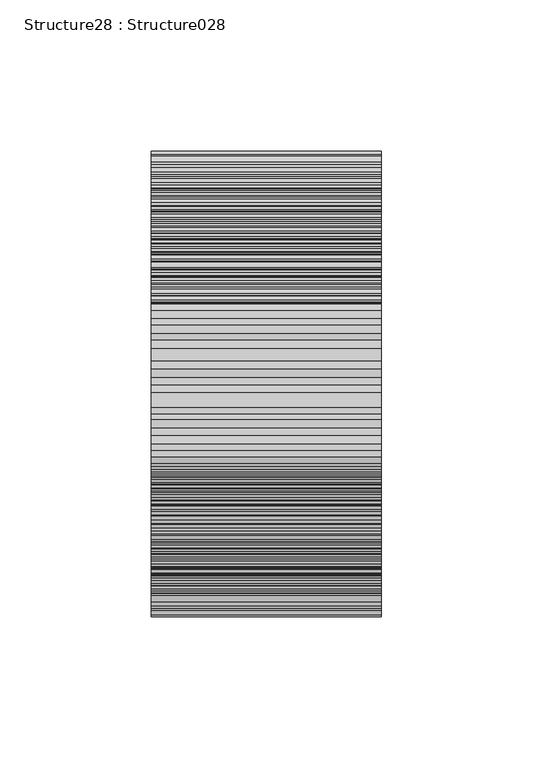
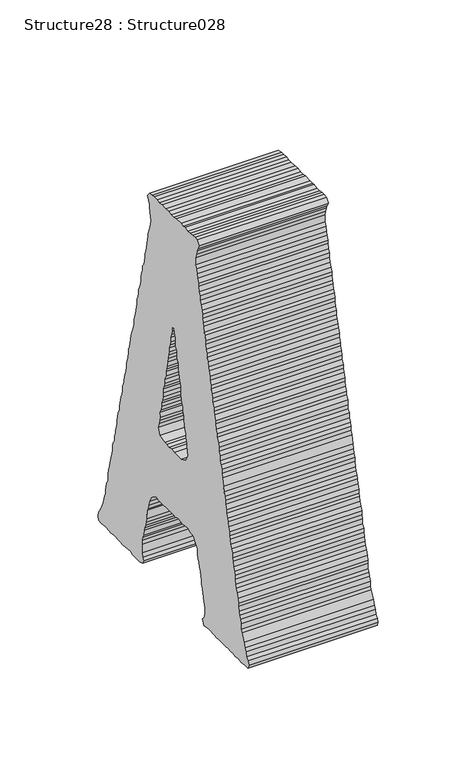
"""IFC4 building model written with IfcOpenShell, lengths in millimetres: proxy geometry, Structure28 : Structure028."""

from ifc_helpers import new_model, si_unit, frame, origin, place, context, project, spatial, polyline, outline, extrude, source, transform, mapped, element, save


def structure28_structure028_1b6d3d0a(model_context):
    return source(origin(), model_context, "Body", "SweptSolid", [
        extrude(outline(polyline([(2.1653931, 0.0), (4.9551582, -1.2360362), (7.1205514, -1.5537289), (9.8959144, -1.859561), (12.3790002, -2.7770574), (14.2258535, -3.09475), (17.0249376, -4.024107), (19.4987044, -4.024107), (22.2740675, -4.9543111), (24.4394606, -5.5778358), (27.2292257, -6.1895001), (29.3937717, -6.8011644), (31.8616083, -7.1069965), (33.7101559, -8.0372006), (36.8159193, -8.3548933), (38.9813125, -8.3548933), (41.7583699, -8.978418), (43.3112516, -9.907775), (46.4093904, -10.5075787), (48.2664099, -11.1311035), (50.7384823, -11.7546283), (53.207166, -11.7546283), (55.371712, -12.3790002), (58.1614771, -13.3083572), (60.6428686, -14.2258535), (63.419926, -14.2258535), (65.2676265, -15.1552105), (68.3750842, -15.7787352), (70.2219375, -15.7787352), (72.7041762, -16.7089393), (75.1770958, -17.0147715), (77.9524588, -17.6382963), (80.1322541, -18.5557927), (84.4621932, -18.5557927), (86.9291825, -17.9441284), (89.4029494, -17.3324641), (91.2591217, -16.3912467), (93.7311941, -15.1552105), (96.2142799, -17.3324641), (96.5226536, -19.4851496), (96.5226536, -21.6624032), (95.9109893, -24.4394606), (95.9109893, -26.9098387), (96.5226536, -29.6987567), (96.2142799, -31.5574705), (96.5226536, -33.7228637), (96.5226536, -38.664467), (95.9109893, -41.1475528), (95.9109893, -43.6187781), (96.5226536, -46.3949883), (96.2142799, -49.1957668), (96.2142799, -53.2080132), (95.9109893, -55.9969312), (96.5226536, -58.1496166), (96.5226536, -60.9503951), (96.2142799, -63.1039277), (95.9109893, -65.8801379), (93.4245148, -67.7515595), (91.2591217, -66.5036627), (89.0945757, -65.8801379), (87.2375562, -65.5861663), (84.4621932, -64.9626415), (79.8094783, -64.0332846), (77.6457795, -64.6568094), (74.8687221, -65.2803342), (69.9135639, -67.1280347), (68.3750842, -67.1280347), (65.5853191, -67.7515595), (63.1166354, -68.3632237), (60.3268703, -68.6809164), (57.8437845, -69.3044412), (55.371712, -70.5277697), (53.5155397, -70.5277697), (50.7384823, -70.834449), (48.2664099, -71.4579738), (46.4093904, -72.7050234), (43.6196253, -72.7050234), (41.1467056, -73.6225198), (38.9813125, -74.234184), (36.5134759, -74.234184), (33.7101559, -74.858556), (31.2507912, -75.7879129), (29.085398, -76.7172698), (27.2292257, -77.0349625), (24.4394606, -77.3407946), (22.2740675, -78.258291), (19.4987044, -78.258291), (17.0249376, -79.1884951), (14.8510727, -79.5061877), (12.0748624, -80.117852), (7.7322156, -81.6588732), (4.9551582, -81.6588732), (2.7906123, -82.282398), (0.3176926, -82.9067699), (-2.4720725, -84.141959), (-4.3282448, -84.4596516), (-6.8020116, -85.0713159), (-9.283403, -85.3890086), (-12.0604605, -86.306505), (-13.9217158, -86.9308769), (-16.7063979, -86.9308769), (-19.4826081, -87.8602338), (-21.3438635, -88.166066), (-24.1344758, -89.0954229), (-26.5929933, -89.4131155), (-29.0752319, -89.7070871), (-30.9322514, -90.3306119), (-33.4136429, -91.260816), (-36.4982268, -91.5666482), (-38.9711464, -92.1901729), (-40.5240281, -93.1195299), (-43.3002383, -93.1195299), (-46.0908506, -93.7311941), (-48.2553966, -94.6613982), (-51.0409258, -95.284923), (-52.9021812, -95.8965873), (-55.0531722, -96.5201121), (-57.5354109, -96.5201121), (-60.6327025, -97.7434406), (-63.1013862, -98.3678125), (-65.2794871, -98.6855052), (-67.7524067, -98.6855052), (-69.6094262, -99.2971695), (-72.6931629, -100.2265264), (-74.5501824, -100.544219), (-77.032421, -101.4617154), (-79.8128671, -101.4617154), (-81.9782603, -102.6977517), (-84.1428062, -103.3212764), (-86.6106428, -103.3212764), (-89.386853, -103.9448012), (-92.1910202, -104.8741582), (-94.3420113, -105.4858224), (-96.2032666, -106.0983339), (-98.9887958, -106.4160265), (-101.4617155, -107.3453834), (-104.2514806, -107.9689082), (-106.7193172, -107.9689082), (-108.8982652, -108.2747403), (-111.0492563, -109.5099294), (-113.8390214, -110.1224408), (-116.311941, -110.7459656), (-118.476487, -110.7459656), (-120.6503519, -111.6753225), (-125.8994818, -113.2163437), (-128.0784298, -114.1465478), (-129.9261303, -115.0759047), (-132.7116595, -116.9346186), (-134.2560694, -117.5462828), (-137.0314325, -118.4764869), (-139.2061446, -117.8529621), (-139.5136711, -114.7700726), (-139.2061446, -112.9223721), (-138.8884519, -110.1224408), (-139.5136711, -107.6512156), (-139.5136711, -104.8741582), (-138.8884519, -102.3919195), (-138.8884519, -100.2265264), (-139.2061446, -97.7434406), (-139.2061446, -95.5907551), (-139.5136711, -92.4960051), (-139.5136711, -90.3306119), (-139.2061446, -87.8602338), (-138.8884519, -85.0713159), (-139.5136711, -82.9067699), (-139.5136711, -75.7879129), (-138.8884519, -73.0108555), (-136.7374609, -71.7638059), (-134.8762055, -72.7050234), (-132.4083689, -73.3166876), (-127.1363652, -73.3166876), (-124.6634456, -73.3166876), (-122.4988996, -72.7050234), (-120.6503519, -71.7638059), (-117.5437413, -71.4579738), (-115.3791954, -70.834449), (-113.2138022, -69.9042449), (-111.0492563, -69.3044412), (-108.5805725, -68.6809164), (-103.0145972, -68.0573916), (-101.4617155, -67.4338668), (-98.9887958, -66.5036627), (-95.8957401, -65.8801379), (-92.8018373, -64.3509773), (-90.9405819, -62.1737236), (-89.0928814, -58.7731414), (-89.7045457, -56.3027633), (-89.7045457, -51.3492994), (-89.386853, -48.2545493), (-89.386853, -41.7710776), (-89.7045457, -38.9702992), (-89.0928814, -36.8176137), (-89.386853, -34.3345279), (-89.7045457, -31.8641498), (-89.386853, -29.6987567), (-89.0928814, -26.6040066), (-89.7045457, -24.7452928), (-90.6372913, -21.0388785), (-92.4943108, -19.1793174), (-95.8957401, -16.7089393), (-98.6719504, -16.7089393), (-101.4617155, -16.0854146), (-103.0145972, -15.1552105), (-106.0991811, -14.8493783), (-107.9697554, -13.6141893), (-110.7459657, -12.9906645), (-112.6029851, -12.6848324), (-115.0759048, -12.6848324), (-117.5437413, -11.4487961), (-120.0302159, -11.1311035), (-122.4988996, -10.8252714), (-124.6634456, -9.907775), (-127.7607372, -8.978418), (-131.7831498, -9.2842502), (-134.8762055, -10.2136071), (-136.4206154, -11.7546283), (-139.5136711, -9.907775), (-139.2061446, -7.1069965), (-138.8884519, -4.6366184), (-138.8884519, 0.3058321), (-139.2061446, 2.7762102), (-139.2061446, 5.259296), (-138.8884519, 7.423842), (-139.2061446, 9.6010957), (-139.2061446, 12.6839852), (-138.8884519, 14.5308385), (-139.2061446, 17.6255886), (-138.8884519, 19.4851496), (-139.5136711, 21.9555277), (-138.8884519, 24.7563062), (-139.5136711, 27.5333636), (-139.2061446, 29.6979095), (-138.8884519, 32.1809953), (-138.8884519, 34.6395129), (-136.4206154, 35.5815775), (-134.2560694, 34.9572056), (-132.7116595, 33.4043239), (-129.9261303, 32.7926596), (-128.0784298, 31.8633027), (-125.2742626, 30.6272664), (-120.6503519, 28.4627205), (-118.7797776, 27.8391957), (-115.7002768, 27.5333636), (-113.2138022, 26.9089916), (-111.0492563, 26.2973273), (-109.2015558, 25.3679704), (-106.0991811, 25.0621383), (-104.2514806, 25.0621383), (-101.4617155, 24.4386135), (-98.6719504, 23.5092566), (-96.5201121, 22.5790525), (-94.3420113, 21.9555277), (-91.565801, 21.6496956), (-89.0928814, 21.355724), (-86.9190164, 21.0380313), (-84.7629423, 19.8028423), (-81.6563317, 19.4851496), (-79.5053406, 19.1784703), (-77.032421, 18.8726382), (-74.858556, 17.9432812), (-72.3856364, 17.0139243), (-69.6094262, 16.4022601), (-68.0556973, 15.7787353), (-65.5827776, 15.7787353), (-62.7980956, 14.8485312), (-60.0074833, 14.5308385), (-58.151311, 13.9191743), (-55.6783914, 13.0016779), (-53.5223172, 12.6839852), (-50.7232331, 11.7546283), (-48.2553966, 11.7546283), (-46.0908506, 11.1302563), (-43.617931, 10.5185921), (-40.8273187, 9.8950673), (-36.1949362, 8.6598782), (-33.7220165, 8.048214), (-31.2397779, 8.048214), (-29.0752319, 7.1180099), (-26.910686, 6.188653), (-23.8125472, 6.188653), (-21.9690826, 4.9534639), (-19.4826081, 4.9534639), (-16.7063979, 4.6476318), (-14.2250064, 3.399735), (-12.0604605, 3.399735), (-9.9094694, 2.164546), (-6.8020116, 1.8468533), (-4.6366185, 1.8468533), (-1.8612554, 0.6235248), (0.0, 0.0), (2.1653931, 0.0)]), holes=[polyline([(-49.7947234, -33.0993389), (-49.7947234, -40.2181959), (-49.5007518, -42.9944061), (-50.1124161, -45.7833241), (-49.5007518, -47.9487172), (-49.7947234, -50.1132632), (-48.2553966, -54.7490344), (-44.2423029, -56.3027633), (-41.1450113, -55.6792385), (-38.9711464, -55.0667271), (-36.8150722, -54.4432023), (-33.7220165, -54.7490344), (-31.5430685, -53.5257059), (-29.0752319, -53.2080132), (-26.910686, -52.9021811), (-24.7452928, -51.9728242), (-22.2639014, -51.6551315), (-19.7909818, -51.6551315), (-17.0147715, -51.3492994), (-15.1535162, -50.4190953), (-12.6848324, -49.8074311), (-10.203441, -49.8074311), (-7.4221477, -48.572242), (-4.6366185, -48.572242), (-2.4720725, -47.6428851), (-0.6099699, -47.3251924), (2.4737668, -47.0185131), (4.9551582, -46.3949883), (7.423842, -45.7833241), (9.5892351, -45.4774919), (12.0748624, -45.4774919), (14.5435462, -44.2423029), (16.7089393, -43.9246102), (19.4987044, -43.9246102), (21.9563748, -42.9944061), (24.1353229, -42.3708814), (26.300716, -42.3708814), (26.6040066, -41.453385), (24.1353229, -40.8417207), (21.6496955, -39.9005033), (19.1810118, -39.5946711), (16.4048016, -39.5946711), (14.5435462, -38.3586349), (11.7537811, -38.0409422), (9.8959144, -38.0409422), (7.423842, -36.8176137), (4.3307863, -36.4999211), (2.1653931, -36.1940889), (0.0, -35.5705641), (-2.4720725, -35.2638848), (-5.2567545, -34.3345279), (-10.203441, -34.0168353), (-12.6848324, -33.4170315), (-15.1535162, -33.0993389), (-16.7063979, -32.169982), (-19.4826081, -32.169982), (-21.9690826, -30.9339457), (-24.4377663, -30.9339457), (-26.5929933, -30.3104209), (-29.3920774, -30.0045888), (-31.2397779, -29.0870924), (-34.0159881, -29.0870924), (-36.8150722, -28.145875), (-38.6627727, -28.145875), (-41.1450113, -27.5333635), (-44.2423029, -26.9098387), (-47.9470229, -28.7693998), (-49.7947234, -33.0993389)])]), frame((-35624.0862846, 277546.3980923, 4122.0266343), z_axis=(1.0, 0.0, 1.354250045437766e-12), x_axis=(-1.354250045437766e-12, 0.0, 1.0)), (0.0, 0.0, 1.0), 76.2),
    ])


if __name__ == "__main__":
    model = new_model("IFC4")
    model_context = context("Model", 3, world=origin())
    ifc_project = project(units=[si_unit("LENGTHUNIT", "METRE", prefix="MILLI")], contexts=[model_context])
    site = spatial("IfcSite", under=ifc_project)
    building = spatial("IfcBuilding", under=site)
    placement = place(None, origin())
    structure28_structure028_shape = structure28_structure028_1b6d3d0a(model_context)
    element("IfcBuildingElementProxy", 1, Name="Structure28 : Structure028", ObjectType="Structure28 : Structure028", at=placement, inside=building, context=model_context, shape_type="MappedRepresentation", body=[
        mapped(structure28_structure028_shape, transform((0.0, 0.0, 0.0), x_axis=(1.0, 0.0, 0.0), y_axis=(0.0, 1.0, 0.0), z_axis=(0.0, 0.0, 1.0))),
    ])
    save(model, "model.ifc")

# Revit data of these elements
# Type "Structure28 : Structure028"
#   NameOverride = "Structure028"
# Element 1 (IfcBuildingElementProxy, "Structure28 : Structure028")
#   Materials on its faces: "BRUSHED ALUMINUM LETTERING"
# Materials
#   "BRUSHED ALUMINUM LETTERING": class "Unassigned", colour RGB 169 181 186, transparency 0, Cost = 0
